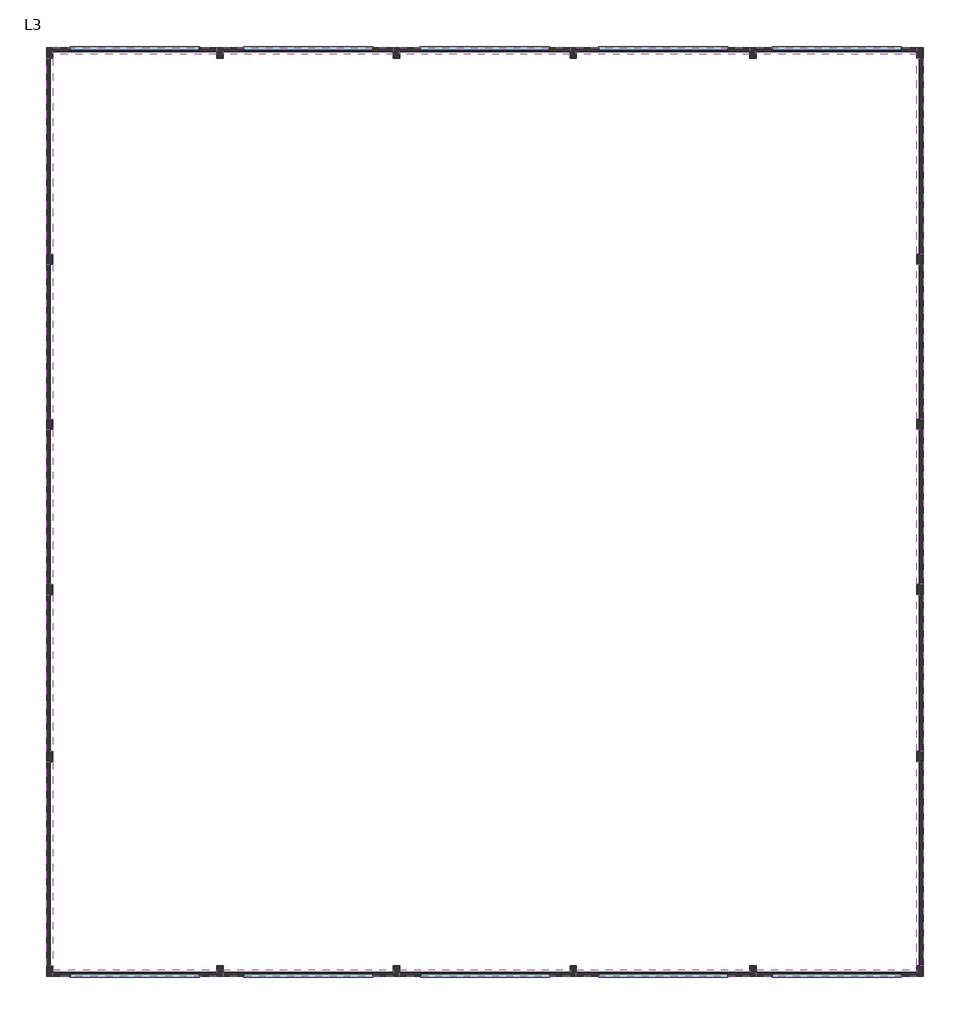
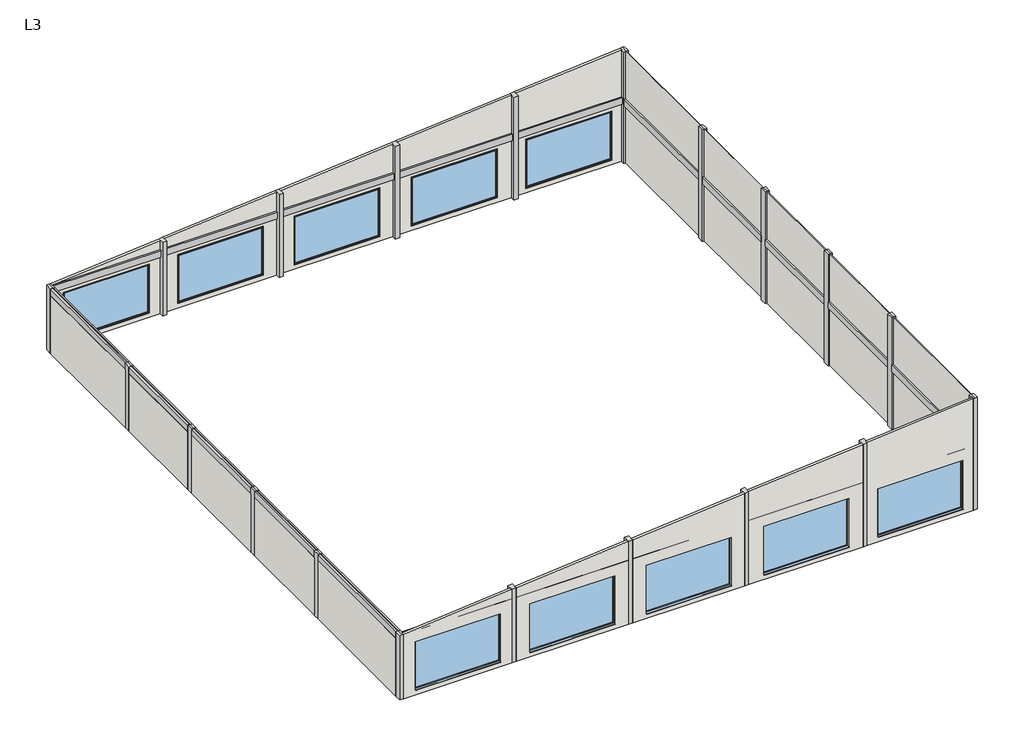
# One storey: 20 beams, 20 columns, 20 walls, 10 windows.
"""IFC4 building model written with IfcOpenShell, lengths in millimetres."""

import ifcopenshell
import ifcopenshell.guid

model = None  # the IFC model being written
_history = None  # IfcOwnerHistory: only IFC2X3 demands one
_inside = {}  # id of a spatial element -> (the spatial element, [elements in it])
_under = {}  # id of a project, library or spatial element -> (it, [spatial elements below it])
_declared = {}  # id of a project -> (the project, [libraries it declares])
_typed = {}  # id of a type object -> (the type object, [elements of that type])
_made_of = {}  # id of a material, layer set ... -> (it, [elements and type objects made of it])


def new_model(schema):
    """Start an empty IFC model of exactly this schema.

    Asked for "IFC4X3", IfcOpenShell would pick the latest addendum, in which some entities
    have other attributes; the version numbers below select the first issue.
    IFC2X3 requires an IfcOwnerHistory on every rooted entity: one is made here for all.
    """
    global model, _history
    if schema == "IFC4X3":
        model = ifcopenshell.file(schema_version=(4, 3, 0, 0))
    else:
        model = ifcopenshell.file(schema=schema)
    _inside.clear()
    _under.clear()
    _declared.clear()
    _typed.clear()
    _made_of.clear()
    _history = None
    if model.schema == "IFC2X3":
        org = make("IfcOrganization", Name="unknown")
        user = make(
            "IfcPersonAndOrganization",
            ThePerson=make("IfcPerson", FamilyName="unknown"),
            TheOrganization=org,
        )
        app = make(
            "IfcApplication",
            ApplicationDeveloper=org,
            Version="unknown",
            ApplicationFullName="unknown",
            ApplicationIdentifier="unknown",
        )
        _history = make(
            "IfcOwnerHistory",
            OwningUser=user,
            OwningApplication=app,
            ChangeAction="ADDED",
            CreationDate=0,
        )
    return model


def make(cls, **values):
    """One entity of the class cls with the attributes given. An attribute that is None is left unset."""
    return model.create_entity(
        cls, **{name: value for name, value in values.items() if value is not None}
    )


def rooted(cls, **values):
    """An entity with a GlobalId (a new one), such as an element, a storey or a relation."""
    return make(cls, GlobalId=ifcopenshell.guid.new(), OwnerHistory=_history, **values)


def si_unit(unit_type, name, prefix=None):
    """IfcSIUnit, for example si_unit("LENGTHUNIT", "METRE", prefix="MILLI")."""
    return make("IfcSIUnit", UnitType=unit_type, Prefix=prefix, Name=name)


def assignment(units):
    """IfcUnitAssignment: the units of a project."""
    return None if units is None else make("IfcUnitAssignment", Units=units)


def point(xyz):
    """IfcCartesianPoint."""
    return None if xyz is None else make("IfcCartesianPoint", Coordinates=xyz)


def direction(xyz):
    """IfcDirection."""
    return None if xyz is None else make("IfcDirection", DirectionRatios=xyz)


def frame(location, z_axis=None, x_axis=None):
    """IfcAxis2Placement3D, a coordinate frame: its origin and axes. An axis left out is left unset."""
    return make(
        "IfcAxis2Placement3D",
        Location=point(location),
        Axis=direction(z_axis),
        RefDirection=direction(x_axis),
    )


def origin():
    """The frame at (0, 0, 0) with its axes left unset."""
    return frame((0.0, 0.0, 0.0))


def place(relative_to, where):
    """IfcLocalPlacement: puts the frame where relative to a parent placement (None: the world)."""
    return make(
        "IfcLocalPlacement", PlacementRelTo=relative_to, RelativePlacement=where
    )


def context(
    kind, dimensions, precision=None, world=None, true_north=None, identifier=None
):
    """IfcGeometricRepresentationContext, for example the 3D "Model" context."""
    return make(
        "IfcGeometricRepresentationContext",
        ContextIdentifier=identifier,
        ContextType=kind,
        CoordinateSpaceDimension=dimensions,
        Precision=precision,
        WorldCoordinateSystem=world,
        TrueNorth=true_north,
    )


def project(units=None, contexts=None):
    """IfcProject with its units and contexts."""
    return rooted(
        "IfcProject",
        Name="project",
        RepresentationContexts=contexts,
        UnitsInContext=assignment(units),
    )


def spatial(cls, under=None, at=None, **own):
    """A site, building, storey or space (cls), placed at a placement, below another one or the project."""
    s = rooted(cls, ObjectPlacement=at, **own)
    if under is not None:
        _under.setdefault(under.id(), (under, []))[1].append(s)
    return s


def polyline(points):
    """IfcPolyline through the points."""
    return make("IfcPolyline", Points=[point(p) for p in points])


def outline(outer, holes=None, kind="AREA"):
    """IfcArbitraryClosedProfileDef: a profile drawn as a closed curve; with holes, ...WithVoids."""
    if holes is None:
        return make("IfcArbitraryClosedProfileDef", ProfileType=kind, OuterCurve=outer)
    return make(
        "IfcArbitraryProfileDefWithVoids",
        ProfileType=kind,
        OuterCurve=outer,
        InnerCurves=holes,
    )


def extrude(swept, where, along, depth):
    """IfcExtrudedAreaSolid: the profile swept, set in the frame where, extruded along a direction by depth."""
    return make(
        "IfcExtrudedAreaSolid",
        SweptArea=swept,
        Position=where,
        ExtrudedDirection=direction(along),
        Depth=depth,
    )


def faces_of(points, faces, orient=None, outer=None):
    """IfcFace entities. A face is a list of loops; a loop is a list of indices into points, from 0.

    orient and outer hold one flag for each loop. By default every Orientation is true, the
    first loop of a face is its IfcFaceOuterBound and the others are IfcFaceBound.
    """
    made = []
    for i, loops in enumerate(faces):
        bounds = []
        for j, loop in enumerate(loops):
            is_outer = j == 0 if outer is None else outer[i][j]
            bounds.append(
                make(
                    "IfcFaceOuterBound" if is_outer else "IfcFaceBound",
                    Bound=make("IfcPolyLoop", Polygon=[points[k] for k in loop]),
                    Orientation=True if orient is None else orient[i][j],
                )
            )
        made.append(make("IfcFace", Bounds=bounds))
    return made


def faceted_brep(points, faces, orient=None, outer=None, voids=None):
    """IfcFacetedBrep: a solid bounded by flat faces; with voids (closed shells), ...WithVoids."""
    shared = [point(p) for p in points]
    hull = make("IfcClosedShell", CfsFaces=faces_of(shared, faces, orient, outer))
    if voids is None:
        return make("IfcFacetedBrep", Outer=hull)
    return make(
        "IfcFacetedBrepWithVoids",
        Outer=hull,
        Voids=[
            make(cls, CfsFaces=faces_of(shared, fs, o, b)) for cls, fs, o, b in voids
        ],
    )


def shape(context_of_items, identifier, shape_type, items):
    """IfcShapeRepresentation: the items that make up one representation, for example the "Body"."""
    return make(
        "IfcShapeRepresentation",
        ContextOfItems=context_of_items,
        RepresentationIdentifier=identifier,
        RepresentationType=shape_type,
        Items=items,
    )


def source(mapping_origin, context_of_items, identifier, shape_type, items):
    """IfcRepresentationMap: a shape defined once, which mapped items show again and again."""
    return make(
        "IfcRepresentationMap",
        MappingOrigin=mapping_origin,
        MappedRepresentation=shape(context_of_items, identifier, shape_type, items),
    )


def transform(
    local_origin,
    x_axis=None,
    y_axis=None,
    z_axis=None,
    scale=None,
    scale2=None,
    scale3=None,
    uniform=True,
):
    """IfcCartesianTransformationOperator3D, or its non-uniform kind. x_axis, y_axis, z_axis: its Axis1, 2, 3."""
    if uniform:
        return make(
            "IfcCartesianTransformationOperator3D",
            Axis1=direction(x_axis),
            Axis2=direction(y_axis),
            LocalOrigin=point(local_origin),
            Scale=scale,
            Axis3=direction(z_axis),
        )
    return make(
        "IfcCartesianTransformationOperator3DnonUniform",
        Axis1=direction(x_axis),
        Axis2=direction(y_axis),
        LocalOrigin=point(local_origin),
        Scale=scale,
        Axis3=direction(z_axis),
        Scale2=scale2,
        Scale3=scale3,
    )


def mapped(mapping_source, mapping_target):
    """IfcMappedItem: shows the shape of a source again, moved by a transform."""
    return make(
        "IfcMappedItem", MappingSource=mapping_source, MappingTarget=mapping_target
    )


def made_of(thing, what):
    """Note that an element or type object is made of a material, layer set ...; save() writes the relation."""
    if what is not None:
        _made_of.setdefault(what.id(), (what, []))[1].append(thing)
    return thing


def element(
    cls,
    number,
    at=None,
    inside=None,
    cuts=None,
    type_object=None,
    material=None,
    context=None,
    identifier="Body",
    shape_type=None,
    held_by="IfcProductDefinitionShape",
    body=None,
    shapes=None,
    **own,
):
    """One element of the class cls, such as IfcWall. Its Tag is "e" and its number.

    at: its placement. inside: the storey or other place that contains it. cuts: it is an
    opening in that element (IfcRelVoidsElement). A single representation is given by context,
    identifier, shape_type and body (its items); several are given by shapes. held_by: the class
    of the entity that holds the representations. save() writes the other relations.
    """
    e = rooted(cls, Tag="e%d" % number, ObjectPlacement=at, **own)
    if body is not None:
        shapes = [shape(context, identifier, shape_type, body)]
    if shapes is not None:
        e.Representation = make(held_by, Representations=shapes)
    if inside is not None:
        _inside.setdefault(inside.id(), (inside, []))[1].append(e)
    if cuts is not None:
        rooted(
            "IfcRelVoidsElement", RelatingBuildingElement=cuts, RelatedOpeningElement=e
        )
    if type_object is not None:
        _typed.setdefault(type_object.id(), (type_object, []))[1].append(e)
    return made_of(e, material)


def aggregate(whole, parts):
    """IfcRelAggregates: a whole, such as a stair, and the parts it consists of."""
    return rooted("IfcRelAggregates", RelatingObject=whole, RelatedObjects=parts)


def save(model, path):
    """Write the relations noted so far, then the file.

    IfcRelAggregates (storeys below a building ...), IfcRelContainedInSpatialStructure (elements
    in a storey), IfcRelDefinesByType, IfcRelAssociatesMaterial and IfcRelDeclares: one each for
    every whole, place, type object, material and project.
    """
    for whole, parts in _under.values():
        aggregate(whole, parts)
    for where, things in _inside.values():
        rooted(
            "IfcRelContainedInSpatialStructure",
            RelatedElements=things,
            RelatingStructure=where,
        )
    for kind, things in _typed.values():
        rooted("IfcRelDefinesByType", RelatedObjects=things, RelatingType=kind)
    for what, things in _made_of.values():
        rooted("IfcRelAssociatesMaterial", RelatedObjects=things, RelatingMaterial=what)
    for by, libraries in _declared.values():
        rooted("IfcRelDeclares", RelatingContext=by, RelatedDefinitions=libraries)
    model.write(path)


def window_5000_x_3000mm_49c9fe68(model_context):
    return source(origin(), model_context, "Body", "SolidModel", [
        extrude(outline(polyline([(125.0, 920.0), (125.0, 900.0), (105.0, 900.0), (105.0, 910.0), (95.0, 910.0), (95.0, 900.0), (-25.0, 900.0), (-25.0, 920.0), (125.0, 920.0)])), frame((-2500.0, 0.0, 0.0), z_axis=(1.0, 0.0, 0.0), x_axis=(0.0, 1.0, 0.0)), (0.0, 0.0, 1.0), 5000.0),
        extrude(outline(polyline([(-2455.0, -49.0), (-2455.0, -35.0), (2455.0, -35.0), (2455.0, -49.0), (-2455.0, -49.0)])), frame((0.0, 0.0, 965.0), z_axis=(0.0, 0.0, 1.0), x_axis=(1.0, 0.0, 0.0)), (0.0, 0.0, 1.0), 2890.0),
        extrude(outline(polyline([(3865.0, -2465.0), (955.0, -2465.0), (955.0, 2465.0), (3865.0, 2465.0), (3865.0, -2465.0)]), holes=[polyline([(3840.0, 2440.0), (980.0, 2440.0), (980.0, -2440.0), (3840.0, -2440.0), (3840.0, 2440.0)])]), frame((0.0, -75.0, 0.0), z_axis=(0.0, 1.0, 0.0), x_axis=(0.0, 0.0, 1.0)), (0.0, 0.0, 1.0), 26.0),
        faceted_brep([(2500.0, -25.0, 3900.0), (2500.0, -75.0, 3900.0), (2500.0, -75.0, 900.0), (2500.0, -25.0, 900.0), (-2500.0, -75.0, 3900.0), (-2500.0, -75.0, 900.0), (-2465.0, -75.0, 3865.0), (2465.0, -75.0, 3865.0), (2465.0, -75.0, 955.0), (-2465.0, -75.0, 955.0), (-2500.0, -25.0, 900.0), (-2500.0, -25.0, 3900.0), (2440.0, -25.0, 3840.0), (-2440.0, -25.0, 3840.0), (-2440.0, -25.0, 980.0), (2440.0, -25.0, 980.0), (2440.0, -35.0, 3840.0), (2440.0, -35.0, 980.0), (-2440.0, -35.0, 980.0), (2465.0, -35.0, 3865.0), (-2465.0, -35.0, 3865.0), (-2465.0, -35.0, 955.0), (2465.0, -35.0, 955.0), (-2440.0, -35.0, 3840.0)], [[[0, 1, 2, 3]], [[2, 1, 4, 5], [6, 7, 8, 9]], [[5, 10, 3, 2]], [[10, 11, 0, 3], [12, 13, 14, 15]], [[16, 12, 15, 17]], [[17, 15, 14, 18]], [[19, 20, 21, 22], [23, 16, 17, 18]], [[7, 19, 22, 8]], [[8, 22, 21, 9]], [[13, 23, 18, 14]], [[20, 6, 9, 21]], [[4, 11, 10, 5]], [[11, 4, 1, 0]], [[23, 13, 12, 16]], [[6, 20, 19, 7]]]),
        extrude(outline(polyline([(3925.0, -2525.0), (875.0, -2525.0), (875.0, 2525.0), (3925.0, 2525.0), (3925.0, -2525.0)]), holes=[polyline([(3890.0, 2490.0), (910.0, 2490.0), (910.0, -2490.0), (3890.0, -2490.0), (3890.0, 2490.0)])]), frame((0.0, -80.0, 0.0), z_axis=(0.0, 1.0, 0.0), x_axis=(0.0, 0.0, 1.0)), (0.0, 0.0, 1.0), 5.0),
    ])


model = new_model("IFC4")

# Units and contexts
model_context = context("Model", 3, world=origin())
ifc_project = project(units=[si_unit("LENGTHUNIT", "METRE", prefix="MILLI")], contexts=[model_context])

# Site, building, storey
site = spatial("IfcSite", under=ifc_project)
building = spatial("IfcBuilding", under=site)
storey = spatial("IfcBuildingStorey", under=building, Name="L3", Elevation=8000.0)

# Beams
placement = place(None, origin())
element("IfcBeam", 1, ObjectType="M_Hormigón-Viga rectangular : 250 x 400mm", at=placement, inside=storey, context=model_context, shape_type="SweptSolid", body=[
    extrude(outline(polyline([(10525.0, 17750.0), (10525.0, 18000.0), (16750.0, 18000.0), (16750.0, 17750.0), (10525.0, 17750.0)])), frame((0.0, 0.0, 11600.0), z_axis=(0.0, 0.0, 1.0), x_axis=(1.0, 0.0, 0.0)), (0.0, 0.0, 1.0), 400.0),
])
element("IfcBeam", 2, ObjectType="M_Hormigón-Viga rectangular : 250 x 400mm", at=placement, inside=storey, context=model_context, shape_type="SweptSolid", body=[
    extrude(outline(polyline([(3550.0, 17750.0), (3550.0, 18000.0), (10275.0, 18000.0), (10275.0, 17750.0), (3550.0, 17750.0)])), frame((0.0, 0.0, 11600.0), z_axis=(0.0, 0.0, 1.0), x_axis=(1.0, 0.0, 0.0)), (0.0, 0.0, 1.0), 400.0),
])
element("IfcBeam", 3, ObjectType="M_Hormigón-Viga rectangular : 250 x 400mm", at=placement, inside=storey, context=model_context, shape_type="SweptSolid", body=[
    extrude(outline(polyline([(-3300.0, 17750.0), (-3300.0, 18000.0), (3300.0, 18000.0), (3300.0, 17750.0), (-3300.0, 17750.0)])), frame((0.0, 0.0, 11600.0), z_axis=(0.0, 0.0, 1.0), x_axis=(1.0, 0.0, 0.0)), (0.0, 0.0, 1.0), 400.0),
])
element("IfcBeam", 4, ObjectType="M_Hormigón-Viga rectangular : 250 x 400mm", at=placement, inside=storey, context=model_context, shape_type="SweptSolid", body=[
    extrude(outline(polyline([(-10150.0, 17750.0), (-10150.0, 18000.0), (-3550.0, 18000.0), (-3550.0, 17750.0), (-10150.0, 17750.0)])), frame((0.0, 0.0, 11600.0), z_axis=(0.0, 0.0, 1.0), x_axis=(1.0, 0.0, 0.0)), (0.0, 0.0, 1.0), 400.0),
])
element("IfcBeam", 5, ObjectType="M_Hormigón-Viga rectangular : 250 x 400mm", at=placement, inside=storey, context=model_context, shape_type="SweptSolid", body=[
    extrude(outline(polyline([(-16750.0, 17750.0), (-16750.0, 18000.0), (-10400.0, 18000.0), (-10400.0, 17750.0), (-16750.0, 17750.0)])), frame((0.0, 0.0, 11600.0), z_axis=(0.0, 0.0, 1.0), x_axis=(1.0, 0.0, 0.0)), (0.0, 0.0, 1.0), 400.0),
])
element("IfcBeam", 6, ObjectType="M_Hormigón-Viga rectangular : 250 x 400mm", at=placement, inside=storey, context=model_context, shape_type="SweptSolid", body=[
    extrude(outline(polyline([(16750.0, -9685.0), (17000.0, -9685.0), (17000.0, -17600.0), (16750.0, -17600.0), (16750.0, -9685.0)])), frame((0.0, 0.0, 11600.0), z_axis=(0.0, 0.0, 1.0), x_axis=(1.0, 0.0, 0.0)), (0.0, 0.0, 1.0), 400.0),
])
element("IfcBeam", 7, ObjectType="M_Hormigón-Viga rectangular : 250 x 400mm", at=placement, inside=storey, context=model_context, shape_type="SweptSolid", body=[
    extrude(outline(polyline([(16750.0, -3200.0), (17000.0, -3200.0), (17000.0, -9285.0), (16750.0, -9285.0), (16750.0, -3200.0)])), frame((0.0, 0.0, 11600.0), z_axis=(0.0, 0.0, 1.0), x_axis=(1.0, 0.0, 0.0)), (0.0, 0.0, 1.0), 400.0),
])
element("IfcBeam", 8, ObjectType="M_Hormigón-Viga rectangular : 250 x 400mm", at=placement, inside=storey, context=model_context, shape_type="SweptSolid", body=[
    extrude(outline(polyline([(16750.0, 3200.0), (17000.0, 3200.0), (17000.0, -2800.0), (16750.0, -2800.0), (16750.0, 3200.0)])), frame((0.0, 0.0, 11600.0), z_axis=(0.0, 0.0, 1.0), x_axis=(1.0, 0.0, 0.0)), (0.0, 0.0, 1.0), 400.0),
])
element("IfcBeam", 9, ObjectType="M_Hormigón-Viga rectangular : 250 x 400mm", at=placement, inside=storey, context=model_context, shape_type="SweptSolid", body=[
    extrude(outline(polyline([(16750.0, 9600.0), (17000.0, 9600.0), (17000.0, 3600.0), (16750.0, 3600.0), (16750.0, 9600.0)])), frame((0.0, 0.0, 11600.0), z_axis=(0.0, 0.0, 1.0), x_axis=(1.0, 0.0, 0.0)), (0.0, 0.0, 1.0), 400.0),
])
element("IfcBeam", 10, ObjectType="M_Hormigón-Viga rectangular : 250 x 400mm", at=placement, inside=storey, context=model_context, shape_type="SweptSolid", body=[
    extrude(outline(polyline([(16750.0, 17600.0), (17000.0, 17600.0), (17000.0, 10000.0), (16750.0, 10000.0), (16750.0, 17600.0)])), frame((0.0, 0.0, 11600.0), z_axis=(0.0, 0.0, 1.0), x_axis=(1.0, 0.0, 0.0)), (0.0, 0.0, 1.0), 400.0),
])
element("IfcBeam", 11, ObjectType="M_Hormigón-Viga rectangular : 250 x 400mm", at=placement, inside=storey, context=model_context, shape_type="SweptSolid", body=[
    extrude(outline(polyline([(10525.0, -18000.0), (10525.0, -17750.0), (16750.0, -17750.0), (16750.0, -18000.0), (10525.0, -18000.0)])), frame((0.0, 0.0, 11600.0), z_axis=(0.0, 0.0, 1.0), x_axis=(1.0, 0.0, 0.0)), (0.0, 0.0, 1.0), 400.0),
])
element("IfcBeam", 12, ObjectType="M_Hormigón-Viga rectangular : 250 x 400mm", at=placement, inside=storey, context=model_context, shape_type="SweptSolid", body=[
    extrude(outline(polyline([(3550.0, -18000.0), (3550.0, -17750.0), (10275.0, -17750.0), (10275.0, -18000.0), (3550.0, -18000.0)])), frame((0.0, 0.0, 11600.0), z_axis=(0.0, 0.0, 1.0), x_axis=(1.0, 0.0, 0.0)), (0.0, 0.0, 1.0), 400.0),
])
element("IfcBeam", 13, ObjectType="M_Hormigón-Viga rectangular : 250 x 400mm", at=placement, inside=storey, context=model_context, shape_type="SweptSolid", body=[
    extrude(outline(polyline([(-3300.0, -18000.0), (-3300.0, -17750.0), (3300.0, -17750.0), (3300.0, -18000.0), (-3300.0, -18000.0)])), frame((0.0, 0.0, 11600.0), z_axis=(0.0, 0.0, 1.0), x_axis=(1.0, 0.0, 0.0)), (0.0, 0.0, 1.0), 400.0),
])
element("IfcBeam", 14, ObjectType="M_Hormigón-Viga rectangular : 250 x 400mm", at=placement, inside=storey, context=model_context, shape_type="SweptSolid", body=[
    extrude(outline(polyline([(-10150.0, -18000.0), (-10150.0, -17750.0), (-3550.0, -17750.0), (-3550.0, -18000.0), (-10150.0, -18000.0)])), frame((0.0, 0.0, 11600.0), z_axis=(0.0, 0.0, 1.0), x_axis=(1.0, 0.0, 0.0)), (0.0, 0.0, 1.0), 400.0),
])
element("IfcBeam", 15, ObjectType="M_Hormigón-Viga rectangular : 250 x 400mm", at=placement, inside=storey, context=model_context, shape_type="SweptSolid", body=[
    extrude(outline(polyline([(-16750.0, -18000.0), (-16750.0, -17750.0), (-10400.0, -17750.0), (-10400.0, -18000.0), (-16750.0, -18000.0)])), frame((0.0, 0.0, 11600.0), z_axis=(0.0, 0.0, 1.0), x_axis=(1.0, 0.0, 0.0)), (0.0, 0.0, 1.0), 400.0),
])
element("IfcBeam", 16, ObjectType="M_Hormigón-Viga rectangular : 250 x 400mm", at=placement, inside=storey, context=model_context, shape_type="SweptSolid", body=[
    extrude(outline(polyline([(-17000.0, -9685.0), (-16750.0, -9685.0), (-16750.0, -17600.0), (-17000.0, -17600.0), (-17000.0, -9685.0)])), frame((0.0, 0.0, 11600.0), z_axis=(0.0, 0.0, 1.0), x_axis=(1.0, 0.0, 0.0)), (0.0, 0.0, 1.0), 400.0),
])
element("IfcBeam", 17, ObjectType="M_Hormigón-Viga rectangular : 250 x 400mm", at=placement, inside=storey, context=model_context, shape_type="SweptSolid", body=[
    extrude(outline(polyline([(-17000.0, -3200.0), (-16750.0, -3200.0), (-16750.0, -9285.0), (-17000.0, -9285.0), (-17000.0, -3200.0)])), frame((0.0, 0.0, 11600.0), z_axis=(0.0, 0.0, 1.0), x_axis=(1.0, 0.0, 0.0)), (0.0, 0.0, 1.0), 400.0),
])
element("IfcBeam", 18, ObjectType="M_Hormigón-Viga rectangular : 250 x 400mm", at=placement, inside=storey, context=model_context, shape_type="SweptSolid", body=[
    extrude(outline(polyline([(-17000.0, 3200.0), (-16750.0, 3200.0), (-16750.0, -2800.0), (-17000.0, -2800.0), (-17000.0, 3200.0)])), frame((0.0, 0.0, 11600.0), z_axis=(0.0, 0.0, 1.0), x_axis=(1.0, 0.0, 0.0)), (0.0, 0.0, 1.0), 400.0),
])
element("IfcBeam", 19, ObjectType="M_Hormigón-Viga rectangular : 250 x 400mm", at=placement, inside=storey, context=model_context, shape_type="SweptSolid", body=[
    extrude(outline(polyline([(-17000.0, 9600.0), (-16750.0, 9600.0), (-16750.0, 3600.0), (-17000.0, 3600.0), (-17000.0, 9600.0)])), frame((0.0, 0.0, 11600.0), z_axis=(0.0, 0.0, 1.0), x_axis=(1.0, 0.0, 0.0)), (0.0, 0.0, 1.0), 400.0),
])
element("IfcBeam", 20, ObjectType="M_Hormigón-Viga rectangular : 250 x 400mm", at=placement, inside=storey, context=model_context, shape_type="SweptSolid", body=[
    extrude(outline(polyline([(-17000.0, 17600.0), (-16750.0, 17600.0), (-16750.0, 10000.0), (-17000.0, 10000.0), (-17000.0, 17600.0)])), frame((0.0, 0.0, 11600.0), z_axis=(0.0, 0.0, 1.0), x_axis=(1.0, 0.0, 0.0)), (0.0, 0.0, 1.0), 400.0),
])

# Columns
element("IfcColumn", 21, ObjectType="M_Hormigón-Rectangular-Pilar : 250 x 400mm", at=placement, inside=storey, context=model_context, shape_type="SweptSolid", body=[
    extrude(outline(polyline([(8000.0, -17000.0), (8000.0, -16750.0), (12010.9360829, -16750.0), (12000.0, -16875.0), (12010.9360829, -16875.0), (12010.9360829, -17000.0), (8000.0, -17000.0)])), frame((0.0, 17600.0, 0.0), z_axis=(0.0, 1.0, 0.0), x_axis=(0.0, 0.0, 1.0)), (0.0, 0.0, 1.0), 400.0),
])
element("IfcColumn", 22, ObjectType="M_Hormigón-Rectangular-Pilar : 250 x 400mm", at=placement, inside=storey, context=model_context, shape_type="SweptSolid", body=[
    extrude(outline(polyline([(8000.0, -10400.0), (8000.0, -10150.0), (12588.3612622, -10150.0), (12566.4890963, -10400.0), (8000.0, -10400.0)])), frame((0.0, 17600.0, 0.0), z_axis=(0.0, 1.0, 0.0), x_axis=(0.0, 0.0, 1.0)), (0.0, 0.0, 1.0), 400.0),
])
element("IfcColumn", 23, ObjectType="M_Hormigón-Rectangular-Pilar : 250 x 400mm", at=placement, inside=storey, context=model_context, shape_type="SweptSolid", body=[
    extrude(outline(polyline([(8000.0, -3550.0), (8000.0, -3300.0), (13187.6586074, -3300.0), (13165.7864415, -3550.0), (8000.0, -3550.0)])), frame((0.0, 17600.0, 0.0), z_axis=(0.0, 1.0, 0.0), x_axis=(0.0, 0.0, 1.0)), (0.0, 0.0, 1.0), 400.0),
])
element("IfcColumn", 24, ObjectType="M_Hormigón-Rectangular-Pilar : 250 x 400mm", at=placement, inside=storey, context=model_context, shape_type="SweptSolid", body=[
    extrude(outline(polyline([(8000.0, 3300.0), (8000.0, 3550.0), (13786.9559525, 3550.0), (13765.0837866, 3300.0), (8000.0, 3300.0)])), frame((0.0, 17600.0, 0.0), z_axis=(0.0, 1.0, 0.0), x_axis=(0.0, 0.0, 1.0)), (0.0, 0.0, 1.0), 400.0),
])
element("IfcColumn", 25, ObjectType="M_Hormigón-Rectangular-Pilar : 250 x 400mm", at=placement, inside=storey, context=model_context, shape_type="SweptSolid", body=[
    extrude(outline(polyline([(8000.0, 10275.0), (8000.0, 10525.0), (14397.1893806, 10525.0), (14375.3172147, 10275.0), (8000.0, 10275.0)])), frame((0.0, 17600.0, 0.0), z_axis=(0.0, 1.0, 0.0), x_axis=(0.0, 0.0, 1.0)), (0.0, 0.0, 1.0), 400.0),
])
element("IfcColumn", 26, ObjectType="M_Hormigón-Rectangular-Pilar : 250 x 400mm", at=placement, inside=storey, context=model_context, shape_type="SweptSolid", body=[
    extrude(outline(polyline([(8000.0, 16750.0), (8000.0, 17000.0), (14952.742394, 17000.0), (14952.742394, 16875.0), (14941.8063111, 16750.0), (8000.0, 16750.0)])), frame((0.0, 17600.0, 0.0), z_axis=(0.0, 1.0, 0.0), x_axis=(0.0, 0.0, 1.0)), (0.0, 0.0, 1.0), 400.0),
])
element("IfcColumn", 27, ObjectType="M_Hormigón-Rectangular-Pilar : 250 x 400mm", at=placement, inside=storey, context=model_context, shape_type="SweptSolid", body=[
    extrude(outline(polyline([(8000.0, -17000.0), (8000.0, -16750.0), (12010.9360829, -16750.0), (12000.0, -16875.0), (12010.9360829, -16875.0), (12010.9360829, -17000.0), (8000.0, -17000.0)])), frame((0.0, 9600.0, 0.0), z_axis=(0.0, 1.0, 0.0), x_axis=(0.0, 0.0, 1.0)), (0.0, 0.0, 1.0), 400.0),
])
element("IfcColumn", 28, ObjectType="M_Hormigón-Rectangular-Pilar : 250 x 400mm", at=placement, inside=storey, context=model_context, shape_type="SweptSolid", body=[
    extrude(outline(polyline([(8000.0, 16750.0), (8000.0, 17000.0), (14952.742394, 17000.0), (14952.742394, 16875.0), (14941.8063111, 16750.0), (8000.0, 16750.0)])), frame((0.0, 9600.0, 0.0), z_axis=(0.0, 1.0, 0.0), x_axis=(0.0, 0.0, 1.0)), (0.0, 0.0, 1.0), 400.0),
])
element("IfcColumn", 29, ObjectType="M_Hormigón-Rectangular-Pilar : 250 x 400mm", at=placement, inside=storey, context=model_context, shape_type="SweptSolid", body=[
    extrude(outline(polyline([(8000.0, -17000.0), (8000.0, -16750.0), (12010.9360829, -16750.0), (12000.0, -16875.0), (12010.9360829, -16875.0), (12010.9360829, -17000.0), (8000.0, -17000.0)])), frame((0.0, 3200.0, 0.0), z_axis=(0.0, 1.0, 0.0), x_axis=(0.0, 0.0, 1.0)), (0.0, 0.0, 1.0), 400.0),
])
element("IfcColumn", 30, ObjectType="M_Hormigón-Rectangular-Pilar : 250 x 400mm", at=placement, inside=storey, context=model_context, shape_type="SweptSolid", body=[
    extrude(outline(polyline([(8000.0, 16750.0), (8000.0, 17000.0), (14952.742394, 17000.0), (14952.742394, 16875.0), (14941.8063111, 16750.0), (8000.0, 16750.0)])), frame((0.0, 3200.0, 0.0), z_axis=(0.0, 1.0, 0.0), x_axis=(0.0, 0.0, 1.0)), (0.0, 0.0, 1.0), 400.0),
])
element("IfcColumn", 31, ObjectType="M_Hormigón-Rectangular-Pilar : 250 x 400mm", at=placement, inside=storey, context=model_context, shape_type="SweptSolid", body=[
    extrude(outline(polyline([(8000.0, -17000.0), (8000.0, -16750.0), (12010.9360829, -16750.0), (12000.0, -16875.0), (12010.9360829, -16875.0), (12010.9360829, -17000.0), (8000.0, -17000.0)])), frame((0.0, -3200.0, 0.0), z_axis=(0.0, 1.0, 0.0), x_axis=(0.0, 0.0, 1.0)), (0.0, 0.0, 1.0), 400.0),
])
element("IfcColumn", 32, ObjectType="M_Hormigón-Rectangular-Pilar : 250 x 400mm", at=placement, inside=storey, context=model_context, shape_type="SweptSolid", body=[
    extrude(outline(polyline([(8000.0, 16750.0), (8000.0, 17000.0), (14952.742394, 17000.0), (14952.742394, 16875.0), (14941.8063111, 16750.0), (8000.0, 16750.0)])), frame((0.0, -3200.0, 0.0), z_axis=(0.0, 1.0, 0.0), x_axis=(0.0, 0.0, 1.0)), (0.0, 0.0, 1.0), 400.0),
])
element("IfcColumn", 33, ObjectType="M_Hormigón-Rectangular-Pilar : 250 x 400mm", at=placement, inside=storey, context=model_context, shape_type="SweptSolid", body=[
    extrude(outline(polyline([(8000.0, -17000.0), (8000.0, -16750.0), (12010.9360829, -16750.0), (12000.0, -16875.0), (12010.9360829, -16875.0), (12010.9360829, -17000.0), (8000.0, -17000.0)])), frame((0.0, -9685.0, 0.0), z_axis=(0.0, 1.0, 0.0), x_axis=(0.0, 0.0, 1.0)), (0.0, 0.0, 1.0), 400.0),
])
element("IfcColumn", 34, ObjectType="M_Hormigón-Rectangular-Pilar : 250 x 400mm", at=placement, inside=storey, context=model_context, shape_type="SweptSolid", body=[
    extrude(outline(polyline([(8000.0, 16750.0), (8000.0, 17000.0), (14952.742394, 17000.0), (14952.742394, 16875.0), (14941.8063111, 16750.0), (8000.0, 16750.0)])), frame((0.0, -9685.0, 0.0), z_axis=(0.0, 1.0, 0.0), x_axis=(0.0, 0.0, 1.0)), (0.0, 0.0, 1.0), 400.0),
])
element("IfcColumn", 35, ObjectType="M_Hormigón-Rectangular-Pilar : 250 x 400mm", at=placement, inside=storey, context=model_context, shape_type="SweptSolid", body=[
    extrude(outline(polyline([(8000.0, -17000.0), (8000.0, -16750.0), (12010.9360829, -16750.0), (12000.0, -16875.0), (12010.9360829, -16875.0), (12010.9360829, -17000.0), (8000.0, -17000.0)])), frame((0.0, -18000.0, 0.0), z_axis=(0.0, 1.0, 0.0), x_axis=(0.0, 0.0, 1.0)), (0.0, 0.0, 1.0), 400.0),
])
element("IfcColumn", 36, ObjectType="M_Hormigón-Rectangular-Pilar : 250 x 400mm", at=placement, inside=storey, context=model_context, shape_type="SweptSolid", body=[
    extrude(outline(polyline([(8000.0, -10400.0), (8000.0, -10150.0), (12588.3612622, -10150.0), (12566.4890963, -10400.0), (8000.0, -10400.0)])), frame((0.0, -18000.0, 0.0), z_axis=(0.0, 1.0, 0.0), x_axis=(0.0, 0.0, 1.0)), (0.0, 0.0, 1.0), 400.0),
])
element("IfcColumn", 37, ObjectType="M_Hormigón-Rectangular-Pilar : 250 x 400mm", at=placement, inside=storey, context=model_context, shape_type="SweptSolid", body=[
    extrude(outline(polyline([(8000.0, -3550.0), (8000.0, -3300.0), (13187.6586074, -3300.0), (13165.7864415, -3550.0), (8000.0, -3550.0)])), frame((0.0, -18000.0, 0.0), z_axis=(0.0, 1.0, 0.0), x_axis=(0.0, 0.0, 1.0)), (0.0, 0.0, 1.0), 400.0),
])
element("IfcColumn", 38, ObjectType="M_Hormigón-Rectangular-Pilar : 250 x 400mm", at=placement, inside=storey, context=model_context, shape_type="SweptSolid", body=[
    extrude(outline(polyline([(8000.0, 3300.0), (8000.0, 3550.0), (13786.9559525, 3550.0), (13765.0837866, 3300.0), (8000.0, 3300.0)])), frame((0.0, -18000.0, 0.0), z_axis=(0.0, 1.0, 0.0), x_axis=(0.0, 0.0, 1.0)), (0.0, 0.0, 1.0), 400.0),
])
element("IfcColumn", 39, ObjectType="M_Hormigón-Rectangular-Pilar : 250 x 400mm", at=placement, inside=storey, context=model_context, shape_type="SweptSolid", body=[
    extrude(outline(polyline([(8000.0, 10275.0), (8000.0, 10525.0), (14397.1893806, 10525.0), (14375.3172147, 10275.0), (8000.0, 10275.0)])), frame((0.0, -18000.0, 0.0), z_axis=(0.0, 1.0, 0.0), x_axis=(0.0, 0.0, 1.0)), (0.0, 0.0, 1.0), 400.0),
])
element("IfcColumn", 40, ObjectType="M_Hormigón-Rectangular-Pilar : 250 x 400mm", at=placement, inside=storey, context=model_context, shape_type="SweptSolid", body=[
    extrude(outline(polyline([(8000.0, 16750.0), (8000.0, 17000.0), (14952.742394, 17000.0), (14952.742394, 16875.0), (14941.8063111, 16750.0), (8000.0, 16750.0)])), frame((0.0, -18000.0, 0.0), z_axis=(0.0, 1.0, 0.0), x_axis=(0.0, 0.0, 1.0)), (0.0, 0.0, 1.0), 400.0),
])

# Walls
element("IfcWall", 41, ObjectType="Genérico - 150 mm DAPC", at=placement, inside=storey, context=model_context, shape_type="SweptSolid", body=[
    extrude(outline(polyline([(8000.0, -16750.0), (8000.0, -10400.0), (12566.4890963, -10400.0), (12010.9360829, -16750.0), (8000.0, -16750.0)]), holes=[polyline([(8300.0, -11075.0), (8300.0, -16075.0), (11300.0, -16075.0), (11300.0, -11075.0), (8300.0, -11075.0)])]), frame((0.0, -18000.0, 0.0), z_axis=(0.0, 1.0, 0.0), x_axis=(0.0, 0.0, 1.0)), (0.0, 0.0, 1.0), 150.0),
])
element("IfcWall", 42, ObjectType="Genérico - 150 mm DAPC", at=placement, inside=storey, context=model_context, shape_type="SweptSolid", body=[
    extrude(outline(polyline([(8000.0, -10150.0), (8000.0, -3550.0), (13165.7864415, -3550.0), (12588.3612622, -10150.0), (8000.0, -10150.0)]), holes=[polyline([(8300.0, -4345.0), (8300.0, -9345.0), (11300.0, -9345.0), (11300.0, -4345.0), (8300.0, -4345.0)])]), frame((0.0, -18000.0, 0.0), z_axis=(0.0, 1.0, 0.0), x_axis=(0.0, 0.0, 1.0)), (0.0, 0.0, 1.0), 150.0),
])
element("IfcWall", 43, ObjectType="Genérico - 150 mm DAPC", at=placement, inside=storey, context=model_context, shape_type="SweptSolid", body=[
    extrude(outline(polyline([(8000.0, -3300.0), (8000.0, 3300.0), (13765.0837866, 3300.0), (13187.6586074, -3300.0), (8000.0, -3300.0)]), holes=[polyline([(8300.0, 2505.0), (8300.0, -2495.0), (11300.0, -2495.0), (11300.0, 2505.0), (8300.0, 2505.0)])]), frame((0.0, -18000.0, 0.0), z_axis=(0.0, 1.0, 0.0), x_axis=(0.0, 0.0, 1.0)), (0.0, 0.0, 1.0), 150.0),
])
element("IfcWall", 44, ObjectType="Genérico - 150 mm DAPC", at=placement, inside=storey, context=model_context, shape_type="SweptSolid", body=[
    extrude(outline(polyline([(8000.0, 3550.0), (8000.0, 10275.0), (14375.3172147, 10275.0), (13786.9559525, 3550.0), (8000.0, 3550.0)]), holes=[polyline([(8300.0, 9412.5), (8300.0, 4412.5), (11300.0, 4412.5), (11300.0, 9412.5), (8300.0, 9412.5)])]), frame((0.0, -18000.0, 0.0), z_axis=(0.0, 1.0, 0.0), x_axis=(0.0, 0.0, 1.0)), (0.0, 0.0, 1.0), 150.0),
])
element("IfcWall", 45, ObjectType="Genérico - 150 mm DAPC", at=placement, inside=storey, context=model_context, shape_type="SweptSolid", body=[
    extrude(outline(polyline([(8000.0, 10525.0), (8000.0, 16750.0), (14941.8063111, 16750.0), (14397.1893806, 10525.0), (8000.0, 10525.0)]), holes=[polyline([(8300.0, 16137.5), (8300.0, 11137.5), (11300.0, 11137.5), (11300.0, 16137.5), (8300.0, 16137.5)])]), frame((0.0, -18000.0, 0.0), z_axis=(0.0, 1.0, 0.0), x_axis=(0.0, 0.0, 1.0)), (0.0, 0.0, 1.0), 150.0),
])
element("IfcWall", 46, ObjectType="Genérico - 150 mm DAPC", at=placement, inside=storey, context=model_context, shape_type="SweptSolid", body=[
    extrude(outline(polyline([(8000.0, 17000.0), (11600.0, 17000.0), (11600.0, 16875.0), (14952.742394, 16875.0), (14950.5551774, 16850.0), (8000.0, 16850.0), (8000.0, 17000.0)])), frame((0.0, -17600.0, 0.0), z_axis=(0.0, 1.0, 0.0), x_axis=(0.0, 0.0, 1.0)), (0.0, 0.0, 1.0), 7930.0),
])
element("IfcWall", 47, ObjectType="Genérico - 150 mm DAPC", at=placement, inside=storey, context=model_context, shape_type="SweptSolid", body=[
    extrude(outline(polyline([(8000.0, 17000.0), (11600.0, 17000.0), (11600.0, 16875.0), (14952.742394, 16875.0), (14950.5551774, 16850.0), (8000.0, 16850.0), (8000.0, 17000.0)])), frame((0.0, -9270.0, 0.0), z_axis=(0.0, 1.0, 0.0), x_axis=(0.0, 0.0, 1.0)), (0.0, 0.0, 1.0), 6070.0),
])
element("IfcWall", 48, ObjectType="Genérico - 150 mm DAPC", at=placement, inside=storey, context=model_context, shape_type="SweptSolid", body=[
    extrude(outline(polyline([(8000.0, 17000.0), (11600.0, 17000.0), (11600.0, 16875.0), (14952.742394, 16875.0), (14950.5551774, 16850.0), (8000.0, 16850.0), (8000.0, 17000.0)])), frame((0.0, -2800.0, 0.0), z_axis=(0.0, 1.0, 0.0), x_axis=(0.0, 0.0, 1.0)), (0.0, 0.0, 1.0), 6000.0),
])
element("IfcWall", 49, ObjectType="Genérico - 150 mm DAPC", at=placement, inside=storey, context=model_context, shape_type="SweptSolid", body=[
    extrude(outline(polyline([(8000.0, 17000.0), (11600.0, 17000.0), (11600.0, 16875.0), (14952.742394, 16875.0), (14950.5551774, 16850.0), (8000.0, 16850.0), (8000.0, 17000.0)])), frame((0.0, 3600.0, 0.0), z_axis=(0.0, 1.0, 0.0), x_axis=(0.0, 0.0, 1.0)), (0.0, 0.0, 1.0), 6000.0),
])
element("IfcWall", 50, ObjectType="Genérico - 150 mm DAPC", at=placement, inside=storey, context=model_context, shape_type="SweptSolid", body=[
    extrude(outline(polyline([(8000.0, 17000.0), (11600.0, 17000.0), (11600.0, 16875.0), (14952.742394, 16875.0), (14950.5551774, 16850.0), (8000.0, 16850.0), (8000.0, 17000.0)])), frame((0.0, 10000.0, 0.0), z_axis=(0.0, 1.0, 0.0), x_axis=(0.0, 0.0, 1.0)), (0.0, 0.0, 1.0), 7600.0),
])
element("IfcWall", 51, ObjectType="Genérico - 150 mm DAPC", at=placement, inside=storey, context=model_context, shape_type="SweptSolid", body=[
    extrude(outline(polyline([(8000.0, 16750.0), (14941.8063111, 16750.0), (14397.1893806, 10525.0), (8000.0, 10525.0), (8000.0, 16750.0)]), holes=[polyline([(8300.0, 11137.5), (11300.0, 11137.5), (11300.0, 16137.5), (8300.0, 16137.5), (8300.0, 11137.5)])]), frame((0.0, 17850.0, 0.0), z_axis=(0.0, 1.0, 0.0), x_axis=(0.0, 0.0, 1.0)), (0.0, 0.0, 1.0), 150.0),
])
element("IfcWall", 52, ObjectType="Genérico - 150 mm DAPC", at=placement, inside=storey, context=model_context, shape_type="SweptSolid", body=[
    extrude(outline(polyline([(8000.0, 10275.0), (14375.3172147, 10275.0), (13786.9559525, 3550.0), (8000.0, 3550.0), (8000.0, 10275.0)]), holes=[polyline([(8300.0, 4412.5), (11300.0, 4412.5), (11300.0, 9412.5), (8300.0, 9412.5), (8300.0, 4412.5)])]), frame((0.0, 17850.0, 0.0), z_axis=(0.0, 1.0, 0.0), x_axis=(0.0, 0.0, 1.0)), (0.0, 0.0, 1.0), 150.0),
])
element("IfcWall", 53, ObjectType="Genérico - 150 mm DAPC", at=placement, inside=storey, context=model_context, shape_type="SweptSolid", body=[
    extrude(outline(polyline([(8000.0, 3300.0), (13765.0837866, 3300.0), (13187.6586074, -3300.0), (8000.0, -3300.0), (8000.0, 3300.0)]), holes=[polyline([(8300.0, -2500.0), (11300.0, -2500.0), (11300.0, 2500.0), (8300.0, 2500.0), (8300.0, -2500.0)])]), frame((0.0, 17850.0, 0.0), z_axis=(0.0, 1.0, 0.0), x_axis=(0.0, 0.0, 1.0)), (0.0, 0.0, 1.0), 150.0),
])
element("IfcWall", 54, ObjectType="Genérico - 150 mm DAPC", at=placement, inside=storey, context=model_context, shape_type="SweptSolid", body=[
    extrude(outline(polyline([(8000.0, -3550.0), (13165.7864415, -3550.0), (12588.3612622, -10150.0), (8000.0, -10150.0), (8000.0, -3550.0)]), holes=[polyline([(8300.0, -9350.0), (11300.0, -9350.0), (11300.0, -4350.0), (8300.0, -4350.0), (8300.0, -9350.0)])]), frame((0.0, 17850.0, 0.0), z_axis=(0.0, 1.0, 0.0), x_axis=(0.0, 0.0, 1.0)), (0.0, 0.0, 1.0), 150.0),
])
element("IfcWall", 55, ObjectType="Genérico - 150 mm DAPC", at=placement, inside=storey, context=model_context, shape_type="SweptSolid", body=[
    extrude(outline(polyline([(8000.0, -10400.0), (12566.4890963, -10400.0), (12010.9360829, -16750.0), (8000.0, -16750.0), (8000.0, -10400.0)]), holes=[polyline([(8300.0, -16075.0), (11300.0, -16075.0), (11300.0, -11075.0), (8300.0, -11075.0), (8300.0, -16075.0)])]), frame((0.0, 17850.0, 0.0), z_axis=(0.0, 1.0, 0.0), x_axis=(0.0, 0.0, 1.0)), (0.0, 0.0, 1.0), 150.0),
])
element("IfcWall", 56, ObjectType="Genérico - 150 mm DAPC", at=placement, inside=storey, context=model_context, shape_type="SweptSolid", body=[
    extrude(outline(polyline([(11600.0, -17000.0), (8000.0, -17000.0), (8000.0, -16850.0), (12002.1872166, -16850.0), (12000.0, -16875.0), (11600.0, -16875.0), (11600.0, -17000.0)])), frame((0.0, 10000.0, 0.0), z_axis=(0.0, 1.0, 0.0), x_axis=(0.0, 0.0, 1.0)), (0.0, 0.0, 1.0), 7600.0),
])
element("IfcWall", 57, ObjectType="Genérico - 150 mm DAPC", at=placement, inside=storey, context=model_context, shape_type="SweptSolid", body=[
    extrude(outline(polyline([(11600.0, -17000.0), (8000.0, -17000.0), (8000.0, -16850.0), (12002.1872166, -16850.0), (12000.0, -16875.0), (11600.0, -16875.0), (11600.0, -17000.0)])), frame((0.0, 3600.0, 0.0), z_axis=(0.0, 1.0, 0.0), x_axis=(0.0, 0.0, 1.0)), (0.0, 0.0, 1.0), 6000.0),
])
element("IfcWall", 58, ObjectType="Genérico - 150 mm DAPC", at=placement, inside=storey, context=model_context, shape_type="SweptSolid", body=[
    extrude(outline(polyline([(11600.0, -17000.0), (8000.0, -17000.0), (8000.0, -16850.0), (12002.1872166, -16850.0), (12000.0, -16875.0), (11600.0, -16875.0), (11600.0, -17000.0)])), frame((0.0, -2800.0, 0.0), z_axis=(0.0, 1.0, 0.0), x_axis=(0.0, 0.0, 1.0)), (0.0, 0.0, 1.0), 6000.0),
])
element("IfcWall", 59, ObjectType="Genérico - 150 mm DAPC", at=placement, inside=storey, context=model_context, shape_type="SweptSolid", body=[
    extrude(outline(polyline([(11600.0, -17000.0), (8000.0, -17000.0), (8000.0, -16850.0), (12002.1872166, -16850.0), (12000.0, -16875.0), (11600.0, -16875.0), (11600.0, -17000.0)])), frame((0.0, -9270.0, 0.0), z_axis=(0.0, 1.0, 0.0), x_axis=(0.0, 0.0, 1.0)), (0.0, 0.0, 1.0), 6070.0),
])
element("IfcWall", 60, ObjectType="Genérico - 150 mm DAPC", at=placement, inside=storey, context=model_context, shape_type="SweptSolid", body=[
    extrude(outline(polyline([(11600.0, -17000.0), (8000.0, -17000.0), (8000.0, -16850.0), (12002.1872166, -16850.0), (12000.0, -16875.0), (11600.0, -16875.0), (11600.0, -17000.0)])), frame((0.0, -17600.0, 0.0), z_axis=(0.0, 1.0, 0.0), x_axis=(0.0, 0.0, 1.0)), (0.0, 0.0, 1.0), 7930.0),
])

# Windows
window_5000_x_3000mm_shape = window_5000_x_3000mm_49c9fe68(model_context)
element("IfcWindow", 61, ObjectType="Ventana simple fija con cubrejuntas interior : 5000 x 3000mm", at=placement, inside=storey, context=model_context, shape_type="MappedRepresentation", body=[
    mapped(window_5000_x_3000mm_shape, transform((-13575.0, -17925.0, 7400.0), x_axis=(-1.0, 0.0, 0.0), y_axis=(0.0, -1.0, 0.0), z_axis=(0.0, 0.0, 1.0))),
])
element("IfcWindow", 62, ObjectType="Ventana simple fija con cubrejuntas interior : 5000 x 3000mm", at=placement, inside=storey, context=model_context, shape_type="MappedRepresentation", body=[
    mapped(window_5000_x_3000mm_shape, transform((-6845.0, -17925.0, 7400.0), x_axis=(-1.0, 0.0, 0.0), y_axis=(0.0, -1.0, 0.0), z_axis=(0.0, 0.0, 1.0))),
])
element("IfcWindow", 63, ObjectType="Ventana simple fija con cubrejuntas interior : 5000 x 3000mm", at=placement, inside=storey, context=model_context, shape_type="MappedRepresentation", body=[
    mapped(window_5000_x_3000mm_shape, transform((5.0, -17925.0, 7400.0), x_axis=(-1.0, 0.0, 0.0), y_axis=(0.0, -1.0, 0.0), z_axis=(0.0, 0.0, 1.0))),
])
element("IfcWindow", 64, ObjectType="Ventana simple fija con cubrejuntas interior : 5000 x 3000mm", at=placement, inside=storey, context=model_context, shape_type="MappedRepresentation", body=[
    mapped(window_5000_x_3000mm_shape, transform((6912.5, -17925.0, 7400.0), x_axis=(-1.0, 0.0, 0.0), y_axis=(0.0, -1.0, 0.0), z_axis=(0.0, 0.0, 1.0))),
])
element("IfcWindow", 65, ObjectType="Ventana simple fija con cubrejuntas interior : 5000 x 3000mm", at=placement, inside=storey, context=model_context, shape_type="MappedRepresentation", body=[
    mapped(window_5000_x_3000mm_shape, transform((13637.5, -17925.0, 7400.0), x_axis=(-1.0, 0.0, 0.0), y_axis=(0.0, -1.0, 0.0), z_axis=(0.0, 0.0, 1.0))),
])
element("IfcWindow", 66, ObjectType="Ventana simple fija con cubrejuntas interior : 5000 x 3000mm", at=placement, inside=storey, context=model_context, shape_type="MappedRepresentation", body=[
    mapped(window_5000_x_3000mm_shape, transform((13637.5, 17925.0, 7400.0), x_axis=(1.0, 0.0, 0.0), y_axis=(0.0, 1.0, 0.0), z_axis=(0.0, 0.0, 1.0))),
])
element("IfcWindow", 67, ObjectType="Ventana simple fija con cubrejuntas interior : 5000 x 3000mm", at=placement, inside=storey, context=model_context, shape_type="MappedRepresentation", body=[
    mapped(window_5000_x_3000mm_shape, transform((6912.5, 17925.0, 7400.0), x_axis=(1.0, 0.0, 0.0), y_axis=(0.0, 1.0, 0.0), z_axis=(0.0, 0.0, 1.0))),
])
element("IfcWindow", 68, ObjectType="Ventana simple fija con cubrejuntas interior : 5000 x 3000mm", at=placement, inside=storey, context=model_context, shape_type="MappedRepresentation", body=[
    mapped(window_5000_x_3000mm_shape, transform((0.0, 17925.0, 7400.0), x_axis=(1.0, 0.0, 0.0), y_axis=(0.0, 1.0, 0.0), z_axis=(0.0, 0.0, 1.0))),
])
element("IfcWindow", 69, ObjectType="Ventana simple fija con cubrejuntas interior : 5000 x 3000mm", at=placement, inside=storey, context=model_context, shape_type="MappedRepresentation", body=[
    mapped(window_5000_x_3000mm_shape, transform((-6850.0, 17925.0, 7400.0), x_axis=(1.0, 0.0, 0.0), y_axis=(0.0, 1.0, 0.0), z_axis=(0.0, 0.0, 1.0))),
])
element("IfcWindow", 70, ObjectType="Ventana simple fija con cubrejuntas interior : 5000 x 3000mm", at=placement, inside=storey, context=model_context, shape_type="MappedRepresentation", body=[
    mapped(window_5000_x_3000mm_shape, transform((-13575.0, 17925.0, 7400.0), x_axis=(1.0, 0.0, 0.0), y_axis=(0.0, 1.0, 0.0), z_axis=(0.0, 0.0, 1.0))),
])

save(model, "model.ifc")

# Revit data of these elements
# Type "M_Hormigón-Viga rectangular : 250 x 400mm"
#   Length [instance default] = 1.524 m
#   b = 0.25 m
#   h = 0.40 m
#   Structural Material [instance default] = Hormigón, Moldeado in situ, gris
# Type "M_Hormigón-Rectangular-Pilar : 250 x 400mm"
#   b = 0.25 m
#   h = 0.40 m
#   Structural Material [instance default] = Hormigón, Moldeado in situ, gris
# Type "Genérico - 150 mm DAPC"
#   Description = "Muro genérico (material por categoría), grosor de 150 mm"
#   Type Mark = "G04"
#   Layers, outside or top first: 0.15 m "Ladrillo, común" (function 1)
# Type "Ventana simple fija con cubrejuntas interior : 5000 x 3000mm"
#   Type Mark = "41"
#   Construction Type Id = "GSP4R"
#   Analytic Construction = "1/8 en cristalera simple Pilkington"
#   Grosor de pared [instance default] = 0.20 m
#   W1 = 4.88 m
#   Visual Light Transmittance = 0.9
#   Anchura de cubrejuntas = 0.035 m
#   Grosor de cubrejuntas = 0.005 m
#   Solar Heat Gain Coefficient = 0.78
#   Grosor de antepecho = 0.02 m
#   Profundidad de antepecho [instance default] = 0.20 m
#   Rough Width = 5.00 m
#   Rough Height = 3.00 m
#   Height = 3.00 m
#   Heat Transfer Coefficient (U) = 3.6886 W/(m²·K)
#   Anchura de marco = 0.06 m
#   Grosor de marco = 0.05 m
#   Anchura de batiente de alzado = 0.50 m
#   Distancia entre antepecho y muro = 0.05 m
#   Altura de antepecho por defecto = 0.90 m
#   Width = 5.00 m
#   Define Thermal Properties by = 1
#   Material de antepecho = none
#   Material de cristalera = Vidrio
#   Material de estructura = none
#   Wall Closure = (empty or 0)
# Elements 1, 11 (IfcBeam, "M_Hormigón-Viga rectangular : 250 x 400mm")
#   Length = 6.475 m
#   Structural Material = Hormigón, Moldeado in situ, gris
#   Phase Created = Nueva construcción
#   Materials on its faces: "Hormigón, Moldeado in situ, gris"
# Elements 2, 12 (IfcBeam, "M_Hormigón-Viga rectangular : 250 x 400mm")
#   Length = 6.975 m
#   Structural Material = Hormigón, Moldeado in situ, gris
#   Phase Created = Nueva construcción
#   Materials on its faces: "Hormigón, Moldeado in situ, gris"
# Elements 3, 4, 13, 14 (IfcBeam, "M_Hormigón-Viga rectangular : 250 x 400mm")
#   Length = 6.85 m
#   Structural Material = Hormigón, Moldeado in situ, gris
#   Phase Created = Nueva construcción
#   Materials on its faces: "Hormigón, Moldeado in situ, gris"
# Elements 5, 15 (IfcBeam, "M_Hormigón-Viga rectangular : 250 x 400mm")
#   Length = 6.60 m
#   Structural Material = Hormigón, Moldeado in situ, gris
#   Phase Created = Nueva construcción
#   Materials on its faces: "Hormigón, Moldeado in situ, gris"
# Elements 6, 16 (IfcBeam, "M_Hormigón-Viga rectangular : 250 x 400mm")
#   Length = 8.33 m
#   Structural Material = Hormigón, Moldeado in situ, gris
#   Phase Created = Nueva construcción
#   Materials on its faces: "Hormigón, Moldeado in situ, gris"
# Elements 7, 17 (IfcBeam, "M_Hormigón-Viga rectangular : 250 x 400mm")
#   Length = 6.47 m
#   Structural Material = Hormigón, Moldeado in situ, gris
#   Phase Created = Nueva construcción
#   Materials on its faces: "Hormigón, Moldeado in situ, gris"
# Elements 8, 9, 18, 19 (IfcBeam, "M_Hormigón-Viga rectangular : 250 x 400mm")
#   Length = 6.40 m
#   Structural Material = Hormigón, Moldeado in situ, gris
#   Phase Created = Nueva construcción
#   Materials on its faces: "Hormigón, Moldeado in situ, gris"
# Elements 10, 20 (IfcBeam, "M_Hormigón-Viga rectangular : 250 x 400mm")
#   Length = 8.00 m
#   Structural Material = Hormigón, Moldeado in situ, gris
#   Phase Created = Nueva construcción
#   Materials on its faces: "Hormigón, Moldeado in situ, gris"
# Elements 21, 22, 23, 24, 25, 26, 27, 28, 29, 30, 31, 32, 33, 34, 35, 36, 37, 38, 39, 40 (IfcColumn, "M_Hormigón-Rectangular-Pilar : 250 x 400mm")
#   Structural Material = Hormigón, Moldeado in situ, gris
#   Phase Created = Nueva construcción
#   Materials on its faces: "Hormigón, Moldeado in situ, gris"
# Elements 41, 42, 43, 44, 45, 46, 47, 48, 49, 50, 51, 52, 53, 54, 55, 56, 57, 58, 59, 60 (IfcWall, "Genérico - 150 mm DAPC")
#   Top Offset = 0.00 m
#   Base Offset = 0.00 m
#   Unconnected Height = 3.60 m
#   wall height = 3.60 m
#   Phase Created = Nueva construcción
#   Base Constraint = L3
#   Materials on its faces: "Ladrillo, común"
# Element 61 (IfcWindow, "Ventana simple fija con cubrejuntas interior : 5000 x 3000mm")
#   Mark = "109"
#   Phase Created = Nueva construcción
#   Materials on its faces: "Vidrio"
# Element 62 (IfcWindow, "Ventana simple fija con cubrejuntas interior : 5000 x 3000mm")
#   Mark = "110"
#   Phase Created = Nueva construcción
#   Materials on its faces: "Vidrio"
# Element 63 (IfcWindow, "Ventana simple fija con cubrejuntas interior : 5000 x 3000mm")
#   Mark = "111"
#   Phase Created = Nueva construcción
#   Materials on its faces: "Vidrio"
# Element 64 (IfcWindow, "Ventana simple fija con cubrejuntas interior : 5000 x 3000mm")
#   Mark = "112"
#   Phase Created = Nueva construcción
#   Materials on its faces: "Vidrio"
# Element 65 (IfcWindow, "Ventana simple fija con cubrejuntas interior : 5000 x 3000mm")
#   Mark = "113"
#   Phase Created = Nueva construcción
#   Materials on its faces: "Vidrio"
# Element 66 (IfcWindow, "Ventana simple fija con cubrejuntas interior : 5000 x 3000mm")
#   Mark = "114"
#   Phase Created = Nueva construcción
#   Materials on its faces: "Vidrio"
# Element 67 (IfcWindow, "Ventana simple fija con cubrejuntas interior : 5000 x 3000mm")
#   Mark = "115"
#   Phase Created = Nueva construcción
#   Materials on its faces: "Vidrio"
# Element 68 (IfcWindow, "Ventana simple fija con cubrejuntas interior : 5000 x 3000mm")
#   Mark = "116"
#   Phase Created = Nueva construcción
#   Materials on its faces: "Vidrio"
# Element 69 (IfcWindow, "Ventana simple fija con cubrejuntas interior : 5000 x 3000mm")
#   Mark = "117"
#   Phase Created = Nueva construcción
#   Materials on its faces: "Vidrio"
# Element 70 (IfcWindow, "Ventana simple fija con cubrejuntas interior : 5000 x 3000mm")
#   Mark = "118"
#   Phase Created = Nueva construcción
#   Materials on its faces: "Vidrio"
# Materials
#   "Hormigón, Moldeado in situ, gris": class "Hormigón", colour RGB 192 192 192, transparency 0, Description = "Hormigón moldeado in situ", Cost = 0
#   "Ladrillo, común": class "Albañilería", colour RGB 121 83 68, transparency 0, Description = "Ladrillo común", Cost = 0
#   "Vidrio": class "Vidrio", colour RGB 245 245 243, transparency 1, Description = "Vidrio de cal sodada", Cost = 0
